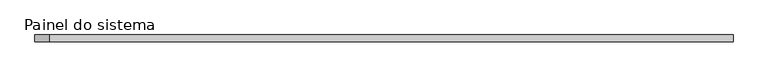
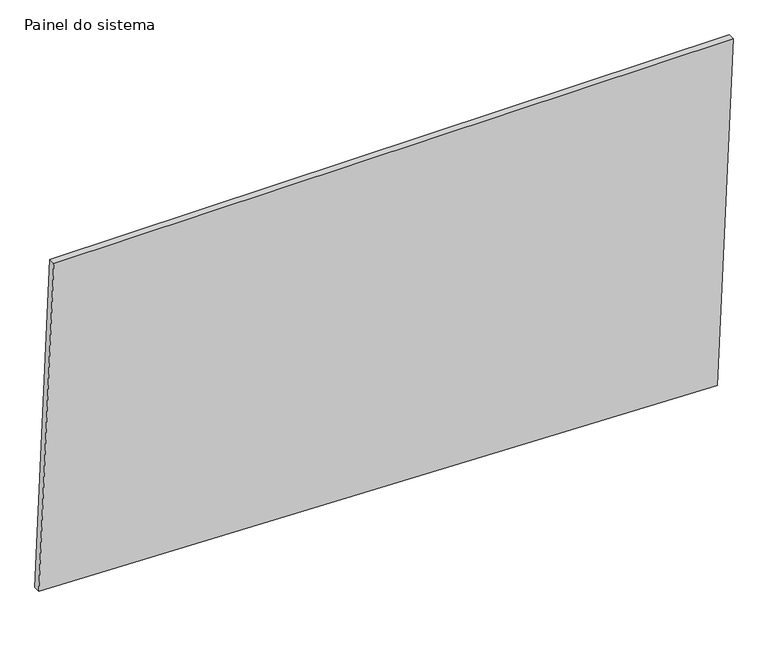
"""IFC4 building model written with IfcOpenShell, lengths in millimetres: plate geometry, Painel do sistema : Envidraçado."""

from ifc_helpers import new_model, si_unit, frame, origin, place, context, project, spatial, polyline, outline, extrude, source, transform, mapped, element, save


def painel_do_sistema_0da9c0cc(model_context):
    return source(origin(), model_context, "Body", "SweptSolid", [
        extrude(outline(polyline([(73.5427954, -1303.2069738), (0.0, 1243.6485277), (1355.5935038, 1303.2069738), (1355.5935038, -1246.8796546), (73.5427954, -1303.2069738)])), frame((0.0, 24.5, 0.0), z_axis=(0.0, 1.0, 0.0), x_axis=(0.0, 0.0, 1.0)), (0.0, 0.0, 1.0), 25.0),
    ])


if __name__ == "__main__":
    model = new_model("IFC4")
    model_context = context("Model", 3, world=origin())
    ifc_project = project(units=[si_unit("LENGTHUNIT", "METRE", prefix="MILLI")], contexts=[model_context])
    site = spatial("IfcSite", under=ifc_project)
    building = spatial("IfcBuilding", under=site)
    placement = place(None, origin())
    painel_do_sistema_shape = painel_do_sistema_0da9c0cc(model_context)
    element("IfcPlate", 1, ObjectType="Painel do sistema : Envidraçado", at=placement, inside=building, context=model_context, shape_type="MappedRepresentation", body=[
        mapped(painel_do_sistema_shape, transform((0.0, 0.0, 0.0), x_axis=(1.0, 0.0, 0.0), y_axis=(0.0, 1.0, 0.0), z_axis=(0.0, 0.0, 1.0))),
    ])
    save(model, "model.ifc")

# Revit data of these elements
# Type "Painel do sistema : Envidraçado"
#   Construction Type Id = "GSP4R"
#   Analytic Construction = "Vidraça única Pilkington 1/8 pol"
#   Visual Light Transmittance = 0.9
#   Solar Heat Gain Coefficient = 0.86
#   Heat Transfer Coefficient (U) = 6.7069 W/(m²·K)
# Element 1 (IfcPlate, "Painel do sistema : Envidraçado")
#   Materials on its faces: "Vidro"
# Materials
#   "Vidro": class "Vidro", colour RGB 0 128 192, transparency 0.9, Description = "Vidro de sílica", Cost = 0
